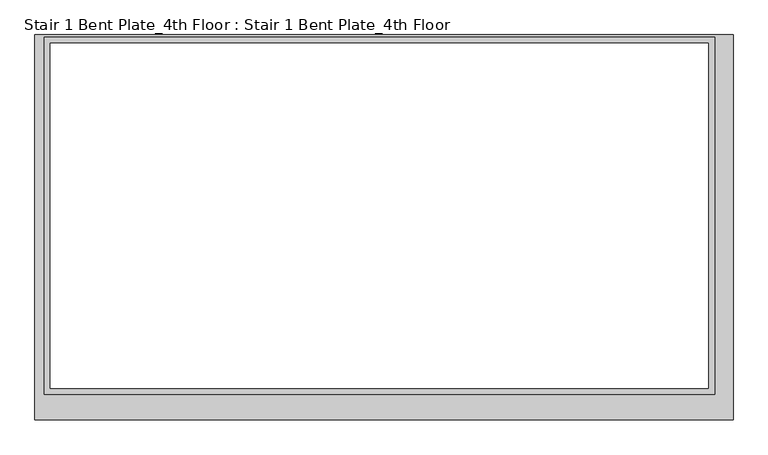
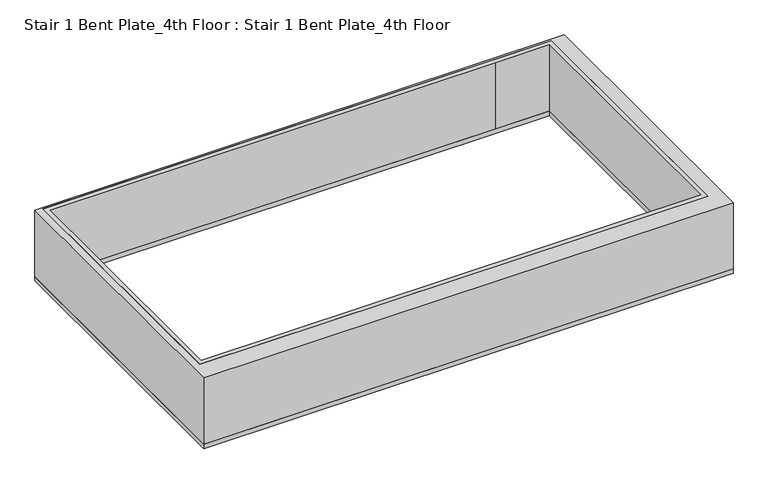
"""IFC4 building model written with IfcOpenShell, lengths in millimetres: proxy geometry, Stair 1 Bent Plate_4th Floor : Stair 1 Bent Plate_4th Floor."""

from ifc_helpers import new_model, si_unit, frame, origin, origin_with_axes, place, context, project, spatial, polyline, outline, extrude, source, transform, mapped, element, save


def stair_1_bent_plate_4th_floor_stair_1_bent_plate_4th_floor_bc49eaa4(model_context):
    return source(origin(), model_context, "Body", "SweptSolid", [
        extrude(outline(polyline([(-266.7, -766.7625), (-266.7, 27.0358273), (1171.575, 27.0358273), (1171.575, -766.7625), (-266.7, -766.7625)]), holes=[polyline([(1133.475, 22.225), (-247.65, 22.225), (-247.65, -714.375), (1133.475, -714.375), (1133.475, 22.225)])]), frame((0.0, 0.0, 12.7), z_axis=(0.0, 0.0, 1.0), x_axis=(1.0, 0.0, 0.0)), (0.0, 0.0, 1.0), 190.5),
        extrude(outline(polyline([(1171.575, -766.7625), (-266.7, -766.7625), (-266.7, 27.0358273), (1171.575, 27.0358273), (1171.575, -766.7625)]), holes=[polyline([(-234.95, 9.525), (-234.95, -701.675), (1120.775, -701.675), (1120.775, 9.525), (-234.95, 9.525)])]), origin_with_axes(), (0.0, 0.0, 1.0), 12.7),
        extrude(outline(polyline([(1133.475, 22.225), (1133.475, -714.375), (-247.65, -714.375), (-247.65, 22.225), (1133.475, 22.225)]), holes=[polyline([(-234.95, -701.675), (1120.775, -701.675), (1120.775, 9.525), (974.725, 9.525), (-234.95, 9.525), (-234.95, -190.5), (-234.95, -701.675)])]), origin_with_axes(), (0.0, 0.0, 1.0), 203.2),
    ])


if __name__ == "__main__":
    model = new_model("IFC4")
    model_context = context("Model", 3, world=origin())
    ifc_project = project(units=[si_unit("LENGTHUNIT", "METRE", prefix="MILLI")], contexts=[model_context])
    site = spatial("IfcSite", under=ifc_project)
    building = spatial("IfcBuilding", under=site)
    placement = place(None, origin())
    stair_1_bent_plate_4th_floor_stair_1_bent_plate_4th_floor_shape = stair_1_bent_plate_4th_floor_stair_1_bent_plate_4th_floor_bc49eaa4(model_context)
    element("IfcBuildingElementProxy", 1, Name="Stair 1 Bent Plate_4th Floor : Stair 1 Bent Plate_4th Floor", ObjectType="Stair 1 Bent Plate_4th Floor : Stair 1 Bent Plate_4th Floor", at=placement, inside=building, context=model_context, shape_type="MappedRepresentation", body=[
        mapped(stair_1_bent_plate_4th_floor_stair_1_bent_plate_4th_floor_shape, transform((0.0, 0.0, 0.0), x_axis=(1.0, 0.0, 0.0), y_axis=(0.0, 1.0, 0.0), z_axis=(0.0, 0.0, 1.0))),
    ])
    save(model, "model.ifc")

# Revit data of these elements
# Element 1 (IfcBuildingElementProxy, "Stair 1 Bent Plate_4th Floor : Stair 1 Bent Plate_4th Floor")
#   Materials on its faces: "Concrete Infill"
# Materials
#   "Concrete Infill": class "Generic", colour RGB 0 255 0, transparency 0, Cost = 0
